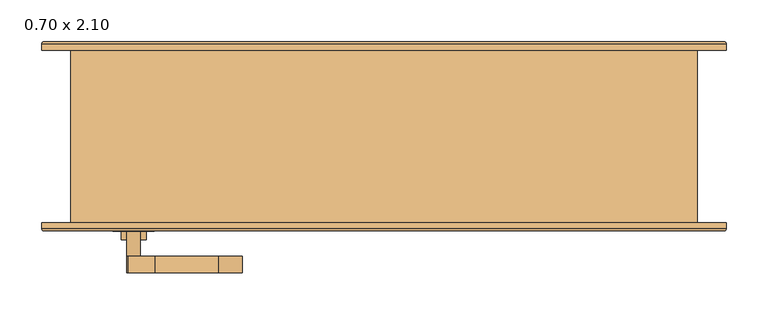
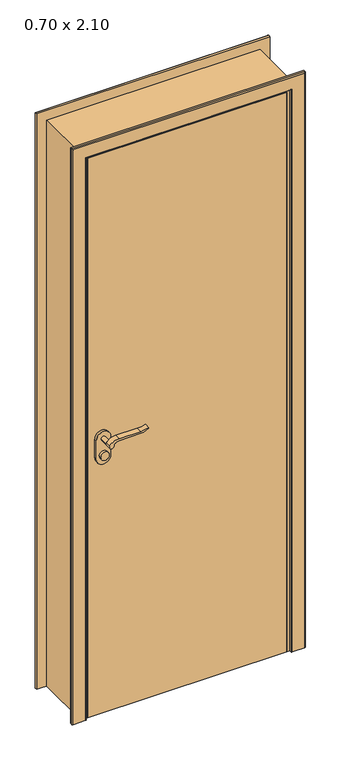
"""IFC4 building model written with IfcOpenShell, lengths in millimetres: door geometry, .CC_ND 300_PORTA SIMPLES DE ABRIR_COM EXTENSÃO : 0.70 x 2.10."""

import ifcopenshell
import ifcopenshell.guid

model = None  # the IFC model being written
_history = None  # IfcOwnerHistory: only IFC2X3 demands one
_inside = {}  # id of a spatial element -> (the spatial element, [elements in it])
_under = {}  # id of a project, library or spatial element -> (it, [spatial elements below it])
_declared = {}  # id of a project -> (the project, [libraries it declares])
_typed = {}  # id of a type object -> (the type object, [elements of that type])
_made_of = {}  # id of a material, layer set ... -> (it, [elements and type objects made of it])


def new_model(schema):
    """Start an empty IFC model of exactly this schema.

    Asked for "IFC4X3", IfcOpenShell would pick the latest addendum, in which some entities
    have other attributes; the version numbers below select the first issue.
    IFC2X3 requires an IfcOwnerHistory on every rooted entity: one is made here for all.
    """
    global model, _history
    if schema == "IFC4X3":
        model = ifcopenshell.file(schema_version=(4, 3, 0, 0))
    else:
        model = ifcopenshell.file(schema=schema)
    _inside.clear()
    _under.clear()
    _declared.clear()
    _typed.clear()
    _made_of.clear()
    _history = None
    if model.schema == "IFC2X3":
        org = make("IfcOrganization", Name="unknown")
        user = make(
            "IfcPersonAndOrganization",
            ThePerson=make("IfcPerson", FamilyName="unknown"),
            TheOrganization=org,
        )
        app = make(
            "IfcApplication",
            ApplicationDeveloper=org,
            Version="unknown",
            ApplicationFullName="unknown",
            ApplicationIdentifier="unknown",
        )
        _history = make(
            "IfcOwnerHistory",
            OwningUser=user,
            OwningApplication=app,
            ChangeAction="ADDED",
            CreationDate=0,
        )
    return model


def make(cls, **values):
    """One entity of the class cls with the attributes given. An attribute that is None is left unset."""
    return model.create_entity(
        cls, **{name: value for name, value in values.items() if value is not None}
    )


def rooted(cls, **values):
    """An entity with a GlobalId (a new one), such as an element, a storey or a relation."""
    return make(cls, GlobalId=ifcopenshell.guid.new(), OwnerHistory=_history, **values)


def si_unit(unit_type, name, prefix=None):
    """IfcSIUnit, for example si_unit("LENGTHUNIT", "METRE", prefix="MILLI")."""
    return make("IfcSIUnit", UnitType=unit_type, Prefix=prefix, Name=name)


def assignment(units):
    """IfcUnitAssignment: the units of a project."""
    return None if units is None else make("IfcUnitAssignment", Units=units)


def point(xyz):
    """IfcCartesianPoint."""
    return None if xyz is None else make("IfcCartesianPoint", Coordinates=xyz)


def direction(xyz):
    """IfcDirection."""
    return None if xyz is None else make("IfcDirection", DirectionRatios=xyz)


def frame(location, z_axis=None, x_axis=None):
    """IfcAxis2Placement3D, a coordinate frame: its origin and axes. An axis left out is left unset."""
    return make(
        "IfcAxis2Placement3D",
        Location=point(location),
        Axis=direction(z_axis),
        RefDirection=direction(x_axis),
    )


def frame_2d(location, x_axis=None):
    """IfcAxis2Placement2D, a coordinate frame in the plane: its origin and x axis."""
    return make(
        "IfcAxis2Placement2D", Location=point(location), RefDirection=direction(x_axis)
    )


def origin():
    """The frame at (0, 0, 0) with its axes left unset."""
    return frame((0.0, 0.0, 0.0))


def origin_with_axes():
    """The frame at (0, 0, 0) with the z axis (0, 0, 1) and the x axis (1, 0, 0) written out."""
    return frame((0.0, 0.0, 0.0), z_axis=(0.0, 0.0, 1.0), x_axis=(1.0, 0.0, 0.0))


def place(relative_to, where):
    """IfcLocalPlacement: puts the frame where relative to a parent placement (None: the world)."""
    return make(
        "IfcLocalPlacement", PlacementRelTo=relative_to, RelativePlacement=where
    )


def context(
    kind, dimensions, precision=None, world=None, true_north=None, identifier=None
):
    """IfcGeometricRepresentationContext, for example the 3D "Model" context."""
    return make(
        "IfcGeometricRepresentationContext",
        ContextIdentifier=identifier,
        ContextType=kind,
        CoordinateSpaceDimension=dimensions,
        Precision=precision,
        WorldCoordinateSystem=world,
        TrueNorth=true_north,
    )


def project(units=None, contexts=None):
    """IfcProject with its units and contexts."""
    return rooted(
        "IfcProject",
        Name="project",
        RepresentationContexts=contexts,
        UnitsInContext=assignment(units),
    )


def spatial(cls, under=None, at=None, **own):
    """A site, building, storey or space (cls), placed at a placement, below another one or the project."""
    s = rooted(cls, ObjectPlacement=at, **own)
    if under is not None:
        _under.setdefault(under.id(), (under, []))[1].append(s)
    return s


def polyline(points):
    """IfcPolyline through the points."""
    return make("IfcPolyline", Points=[point(p) for p in points])


def circle_curve(where, radius):
    """IfcCircle in the frame where."""
    return make("IfcCircle", Position=where, Radius=radius)


def ellipse_curve(where, semi_axis1, semi_axis2):
    """IfcEllipse in the frame where."""
    return make(
        "IfcEllipse", Position=where, SemiAxis1=semi_axis1, SemiAxis2=semi_axis2
    )


def trimmed(basis, trim1, trim2, sense, master):
    """IfcTrimmedCurve: the piece of a basis curve between two trims."""
    return make(
        "IfcTrimmedCurve",
        BasisCurve=basis,
        Trim1=trim1,
        Trim2=trim2,
        SenseAgreement=sense,
        MasterRepresentation=master,
    )


def segment(curve, same_sense, transition):
    """IfcCompositeCurveSegment."""
    return make(
        "IfcCompositeCurveSegment",
        Transition=transition,
        SameSense=same_sense,
        ParentCurve=curve,
    )


def composite_curve(segments, self_intersect=None):
    """IfcCompositeCurve: segments joined end to end."""
    return make("IfcCompositeCurve", Segments=segments, SelfIntersect=self_intersect)


def outline(outer, holes=None, kind="AREA"):
    """IfcArbitraryClosedProfileDef: a profile drawn as a closed curve; with holes, ...WithVoids."""
    if holes is None:
        return make("IfcArbitraryClosedProfileDef", ProfileType=kind, OuterCurve=outer)
    return make(
        "IfcArbitraryProfileDefWithVoids",
        ProfileType=kind,
        OuterCurve=outer,
        InnerCurves=holes,
    )


def extrude(swept, where, along, depth):
    """IfcExtrudedAreaSolid: the profile swept, set in the frame where, extruded along a direction by depth."""
    return make(
        "IfcExtrudedAreaSolid",
        SweptArea=swept,
        Position=where,
        ExtrudedDirection=direction(along),
        Depth=depth,
    )


def faces_of(points, faces, orient=None, outer=None):
    """IfcFace entities. A face is a list of loops; a loop is a list of indices into points, from 0.

    orient and outer hold one flag for each loop. By default every Orientation is true, the
    first loop of a face is its IfcFaceOuterBound and the others are IfcFaceBound.
    """
    made = []
    for i, loops in enumerate(faces):
        bounds = []
        for j, loop in enumerate(loops):
            is_outer = j == 0 if outer is None else outer[i][j]
            bounds.append(
                make(
                    "IfcFaceOuterBound" if is_outer else "IfcFaceBound",
                    Bound=make("IfcPolyLoop", Polygon=[points[k] for k in loop]),
                    Orientation=True if orient is None else orient[i][j],
                )
            )
        made.append(make("IfcFace", Bounds=bounds))
    return made


def faceted_brep(points, faces, orient=None, outer=None, voids=None):
    """IfcFacetedBrep: a solid bounded by flat faces; with voids (closed shells), ...WithVoids."""
    shared = [point(p) for p in points]
    hull = make("IfcClosedShell", CfsFaces=faces_of(shared, faces, orient, outer))
    if voids is None:
        return make("IfcFacetedBrep", Outer=hull)
    return make(
        "IfcFacetedBrepWithVoids",
        Outer=hull,
        Voids=[
            make(cls, CfsFaces=faces_of(shared, fs, o, b)) for cls, fs, o, b in voids
        ],
    )


def shape(context_of_items, identifier, shape_type, items):
    """IfcShapeRepresentation: the items that make up one representation, for example the "Body"."""
    return make(
        "IfcShapeRepresentation",
        ContextOfItems=context_of_items,
        RepresentationIdentifier=identifier,
        RepresentationType=shape_type,
        Items=items,
    )


def source(mapping_origin, context_of_items, identifier, shape_type, items):
    """IfcRepresentationMap: a shape defined once, which mapped items show again and again."""
    return make(
        "IfcRepresentationMap",
        MappingOrigin=mapping_origin,
        MappedRepresentation=shape(context_of_items, identifier, shape_type, items),
    )


def transform(
    local_origin,
    x_axis=None,
    y_axis=None,
    z_axis=None,
    scale=None,
    scale2=None,
    scale3=None,
    uniform=True,
):
    """IfcCartesianTransformationOperator3D, or its non-uniform kind. x_axis, y_axis, z_axis: its Axis1, 2, 3."""
    if uniform:
        return make(
            "IfcCartesianTransformationOperator3D",
            Axis1=direction(x_axis),
            Axis2=direction(y_axis),
            LocalOrigin=point(local_origin),
            Scale=scale,
            Axis3=direction(z_axis),
        )
    return make(
        "IfcCartesianTransformationOperator3DnonUniform",
        Axis1=direction(x_axis),
        Axis2=direction(y_axis),
        LocalOrigin=point(local_origin),
        Scale=scale,
        Axis3=direction(z_axis),
        Scale2=scale2,
        Scale3=scale3,
    )


def mapped(mapping_source, mapping_target):
    """IfcMappedItem: shows the shape of a source again, moved by a transform."""
    return make(
        "IfcMappedItem", MappingSource=mapping_source, MappingTarget=mapping_target
    )


def made_of(thing, what):
    """Note that an element or type object is made of a material, layer set ...; save() writes the relation."""
    if what is not None:
        _made_of.setdefault(what.id(), (what, []))[1].append(thing)
    return thing


def element(
    cls,
    number,
    at=None,
    inside=None,
    cuts=None,
    type_object=None,
    material=None,
    context=None,
    identifier="Body",
    shape_type=None,
    held_by="IfcProductDefinitionShape",
    body=None,
    shapes=None,
    **own,
):
    """One element of the class cls, such as IfcWall. Its Tag is "e" and its number.

    at: its placement. inside: the storey or other place that contains it. cuts: it is an
    opening in that element (IfcRelVoidsElement). A single representation is given by context,
    identifier, shape_type and body (its items); several are given by shapes. held_by: the class
    of the entity that holds the representations. save() writes the other relations.
    """
    e = rooted(cls, Tag="e%d" % number, ObjectPlacement=at, **own)
    if body is not None:
        shapes = [shape(context, identifier, shape_type, body)]
    if shapes is not None:
        e.Representation = make(held_by, Representations=shapes)
    if inside is not None:
        _inside.setdefault(inside.id(), (inside, []))[1].append(e)
    if cuts is not None:
        rooted(
            "IfcRelVoidsElement", RelatingBuildingElement=cuts, RelatedOpeningElement=e
        )
    if type_object is not None:
        _typed.setdefault(type_object.id(), (type_object, []))[1].append(e)
    return made_of(e, material)


def aggregate(whole, parts):
    """IfcRelAggregates: a whole, such as a stair, and the parts it consists of."""
    return rooted("IfcRelAggregates", RelatingObject=whole, RelatedObjects=parts)


def save(model, path):
    """Write the relations noted so far, then the file.

    IfcRelAggregates (storeys below a building ...), IfcRelContainedInSpatialStructure (elements
    in a storey), IfcRelDefinesByType, IfcRelAssociatesMaterial and IfcRelDeclares: one each for
    every whole, place, type object, material and project.
    """
    for whole, parts in _under.values():
        aggregate(whole, parts)
    for where, things in _inside.values():
        rooted(
            "IfcRelContainedInSpatialStructure",
            RelatedElements=things,
            RelatingStructure=where,
        )
    for kind, things in _typed.values():
        rooted("IfcRelDefinesByType", RelatedObjects=things, RelatingType=kind)
    for what, things in _made_of.values():
        rooted("IfcRelAssociatesMaterial", RelatedObjects=things, RelatingMaterial=what)
    for by, libraries in _declared.values():
        rooted("IfcRelDeclares", RelatingContext=by, RelatedDefinitions=libraries)
    model.write(path)


def plane_surface(at):
    """IfcPlane: the flat surface through the origin of the frame at, square to its z axis."""
    return make("IfcPlane", Position=at)


def cylinder_surface(at, radius):
    """IfcCylindricalSurface: all points at the distance radius from the z axis of the frame at."""
    return make("IfcCylindricalSurface", Position=at, Radius=radius)


def advanced_brep(points, edges, surfaces, faces):
    """IfcAdvancedBrep: a solid bounded by faces that lie on surfaces and meet in shared edges.

    An edge is (start, end): straight between two places in points (the first is 0);
    or (start, end, curve); or (start, end, curve, False) where it runs against its curve.
    A face is (place in surfaces, loops), or (place, loops, False) where it looks against
    its surface's normal. A loop lists edges by number (the first is 1), with a minus sign
    where the edge is run from its end to its start. The first loop is the outer one.
    """
    corners = [point(p) for p in points]
    vertices = [make("IfcVertexPoint", VertexGeometry=c) for c in corners]
    made = []
    for start, end, *more in edges:
        made.append(
            make(
                "IfcEdgeCurve",
                EdgeStart=vertices[start],
                EdgeEnd=vertices[end],
                EdgeGeometry=more[0] if more else make("IfcPolyline", Points=[corners[start], corners[end]]),
                SameSense=more[1] if len(more) > 1 else True,
            )
        )
    hull = []
    for where, loops, *sense in faces:
        bounds = []
        for j, loop in enumerate(loops):
            ring = [make("IfcOrientedEdge", EdgeElement=made[abs(k) - 1], Orientation=k > 0) for k in loop]
            bounds.append(
                make(
                    "IfcFaceOuterBound" if j == 0 else "IfcFaceBound",
                    Bound=make("IfcEdgeLoop", EdgeList=ring),
                    Orientation=True,
                )
            )
        hull.append(make("IfcAdvancedFace", Bounds=bounds, FaceSurface=surfaces[where], SameSense=sense[0] if sense else True))
    return make("IfcAdvancedBrep", Outer=make("IfcClosedShell", CfsFaces=hull))


def door_0_70_x_2_10_d125a7d3(model_context):
    return source(origin(), model_context, "Body", "SolidModel", [
        extrude(outline(composite_curve([segment(trimmed(circle_curve(frame_2d((964.5, -300.0)), 15.0), [point((964.5, -285.0))], [point((964.5, -315.0))], False, "CARTESIAN"), True, "CONTINUOUS"), segment(trimmed(circle_curve(frame_2d((964.5, -300.0)), 15.0), [point((964.5, -315.0))], [point((964.5, -285.0))], False, "CARTESIAN"), True, "CONTINUOUS")], self_intersect=False)), frame((0.0, -120.7, 0.0), z_axis=(0.0, 1.0, 0.0), x_axis=(0.0, 0.0, 1.0)), (0.0, 0.0, 1.0), 10.0),
        extrude(outline(composite_curve([segment(trimmed(circle_curve(frame_2d((964.5, -300.0)), 15.0), [point((964.5, -285.0))], [point((964.5, -315.0))], False, "CARTESIAN"), True, "CONTINUOUS"), segment(trimmed(circle_curve(frame_2d((964.5, -300.0)), 15.0), [point((964.5, -315.0))], [point((964.5, -285.0))], False, "CARTESIAN"), True, "CONTINUOUS")], self_intersect=False)), frame((0.0, -60.7, 0.0), z_axis=(0.0, 1.0, 0.0), x_axis=(0.0, 0.0, 1.0)), (0.0, 0.0, 1.0), 10.0),
        extrude(outline(composite_curve([segment(trimmed(circle_curve(frame_2d((1024.5, -300.0)), 8.0), [point((1029.1523287, -306.5081363))], [point((1024.5, -292.0))], False, "CARTESIAN"), True, "CONTINUOUS"), segment(trimmed(circle_curve(frame_2d((1019.3738613, -274.6138099)), 18.1261387), [point((1024.5, -292.0))], [point((1037.5, -274.6138099))], True, "CARTESIAN"), True, "CONTINUOUS"), segment(polyline([(1037.5, -274.6138099), (1037.5, -198.3564091)]), True, "CONTINUOUS"), segment(trimmed(circle_curve(frame_2d((1096.7709207, -201.9396612)), 59.3791355), [point((1037.5, -198.3564091))], [point((1046.7135558, -170.0))], False, "CARTESIAN"), True, "CONTINUOUS"), segment(polyline([(1046.7135558, -170.0), (1049.5, -170.0)]), True, "CONTINUOUS"), segment(trimmed(circle_curve(frame_2d((1127.7850638, -198.4227909)), 83.2850902), [point((1049.5, -170.0))], [point((1044.5, -198.3564091))], True, "CARTESIAN"), True, "CONTINUOUS"), segment(polyline([(1044.5, -198.3564091), (1044.5, -274.6325667)]), True, "CONTINUOUS"), segment(trimmed(circle_curve(frame_2d((1007.2555521, -276.3324871)), 37.2832219), [point((1044.5, -274.6325667))], [point((1029.1523287, -306.5081363))], False, "CARTESIAN"), True, "CONTINUOUS")], self_intersect=False)), frame((0.0, -160.7, 0.0), z_axis=(0.0, 1.0, 0.0), x_axis=(0.0, 0.0, 1.0)), (0.0, 0.0, 1.0), 20.0),
        extrude(outline(composite_curve([segment(trimmed(circle_curve(frame_2d((1019.3738682, -274.6138122)), 18.1261318), [point((1024.4999903, -292.0))], [point((1037.5, -274.6138122))], True, "CARTESIAN"), True, "CONTINUOUS"), segment(polyline([(1037.5, -274.6138122), (1037.5, -198.3564091)]), True, "CONTINUOUS"), segment(trimmed(circle_curve(frame_2d((1096.7709207, -201.9396612)), 59.3791355), [point((1037.5, -198.3564091))], [point((1046.7135558, -170.0))], False, "CARTESIAN"), True, "CONTINUOUS"), segment(polyline([(1046.7135558, -170.0), (1049.5, -170.0)]), True, "CONTINUOUS"), segment(trimmed(circle_curve(frame_2d((1127.7850638, -198.4227909)), 83.2850902), [point((1049.5, -170.0))], [point((1044.5, -198.3564091))], True, "CARTESIAN"), True, "CONTINUOUS"), segment(polyline([(1044.5, -198.3564091), (1044.5, -274.6325667)]), True, "CONTINUOUS"), segment(trimmed(circle_curve(frame_2d((1007.2555521, -276.3324871)), 37.2832219), [point((1044.5, -274.6325667))], [point((1029.1523287, -306.5081363))], False, "CARTESIAN"), True, "CONTINUOUS"), segment(trimmed(circle_curve(frame_2d((1024.5, -300.0)), 8.0), [point((1029.1523287, -306.5081363))], [point((1024.4999903, -292.0))], False, "CARTESIAN"), True, "CONTINUOUS")], self_intersect=False)), frame((0.0, -30.7, 0.0), z_axis=(0.0, 1.0, 0.0), x_axis=(0.0, 0.0, 1.0)), (0.0, 0.0, 1.0), 20.0),
        extrude(outline(composite_curve([segment(trimmed(circle_curve(frame_2d((1024.5, -300.0)), 8.0), [point((1024.5, -292.0))], [point((1024.5, -308.0))], False, "CARTESIAN"), True, "CONTINUOUS"), segment(trimmed(circle_curve(frame_2d((1024.5, -300.0)), 8.0), [point((1024.5, -308.0))], [point((1024.5, -292.0))], False, "CARTESIAN"), True, "CONTINUOUS")], self_intersect=False)), frame((0.0, -140.7, 0.0), z_axis=(0.0, 1.0, 0.0), x_axis=(0.0, 0.0, 1.0)), (0.0, 0.0, 1.0), 30.0),
        extrude(outline(composite_curve([segment(trimmed(circle_curve(frame_2d((1024.5, -300.0)), 8.0), [point((1024.5, -292.0))], [point((1024.5, -308.0))], False, "CARTESIAN"), True, "CONTINUOUS"), segment(trimmed(circle_curve(frame_2d((1024.5, -300.0)), 8.0), [point((1024.5, -308.0))], [point((1024.5, -292.0))], False, "CARTESIAN"), True, "CONTINUOUS")], self_intersect=False)), frame((0.0, -60.7, 0.0), z_axis=(0.0, 1.0, 0.0), x_axis=(0.0, 0.0, 1.0)), (0.0, 0.0, 1.0), 30.0),
        extrude(outline(composite_curve([segment(trimmed(circle_curve(frame_2d((954.5, -300.0)), 25.0), [point((954.5, -325.0))], [point((954.5, -275.0))], False, "CARTESIAN"), True, "CONTINUOUS"), segment(polyline([(954.5, -275.0), (1024.5, -275.0)]), True, "CONTINUOUS"), segment(trimmed(circle_curve(frame_2d((1024.5, -300.0)), 25.0), [point((1024.5, -275.0))], [point((1024.5, -325.0))], False, "CARTESIAN"), True, "CONTINUOUS"), segment(polyline([(1024.5, -325.0), (954.5, -325.0)]), True, "CONTINUOUS")], self_intersect=False)), frame((0.0, -110.7, 0.0), z_axis=(0.0, 1.0, 0.0), x_axis=(0.0, 0.0, 1.0)), (0.0, 0.0, 1.0), 10.0),
        extrude(outline(composite_curve([segment(trimmed(circle_curve(frame_2d((954.5, -300.0)), 25.0), [point((954.5, -325.0))], [point((954.5, -275.0))], False, "CARTESIAN"), True, "CONTINUOUS"), segment(polyline([(954.5, -275.0), (1024.5, -275.0)]), True, "CONTINUOUS"), segment(trimmed(circle_curve(frame_2d((1024.5, -300.0)), 25.0), [point((1024.5, -275.0))], [point((1024.5, -325.0))], False, "CARTESIAN"), True, "CONTINUOUS"), segment(polyline([(1024.5, -325.0), (954.5, -325.0)]), True, "CONTINUOUS")], self_intersect=False)), frame((0.0, -70.7, 0.0), z_axis=(0.0, 1.0, 0.0), x_axis=(0.0, 0.0, 1.0)), (0.0, 0.0, 1.0), 10.0),
        advanced_brep(
        [(-410.0, -100.7, 0.0), (-360.0, -100.7, 0.0), (-360.0, -107.7, 0.0), (-363.0, -110.7, 0.0), (-407.0, -110.7, 0.0), (-410.0, -107.7, 0.0), (-410.0, -100.7, 2135.0), (410.0, -100.7, 2135.0), (410.0, -100.7, 0.0), (360.0, -100.7, 0.0), (360.0, -100.7, 2085.0), (-360.0, -100.7, 2085.0), (-360.0, -107.7, 2085.0), (-363.0, -110.7, 2088.0), (363.0, -110.7, 2088.0), (363.0, -110.7, 0.0), (407.0, -110.7, 0.0), (407.0, -110.7, 2132.0), (-407.0, -110.7, 2132.0), (-410.0, -107.7, 2135.0), (410.0, -107.7, 2135.0), (410.0, -107.7, 0.0), (360.0, -107.7, 0.0), (360.0, -107.7, 2085.0)],
        [
            (0, 1),
            (1, 2),
            (2, 3, circle_curve(frame((-363.0, -107.7, 0.0), z_axis=(0.0, 0.0, -1.0), x_axis=(1.0, 0.0, 0.0)), 3.0)),
            (3, 4),
            (4, 5, circle_curve(frame((-407.0, -107.7, 0.0), z_axis=(0.0, 0.0, -1.0), x_axis=(1.0, 0.0, 0.0)), 3.0)),
            (5, 0),
            (0, 6),
            (6, 7),
            (7, 8),
            (8, 9),
            (9, 10),
            (10, 11),
            (11, 1),
            (11, 12),
            (12, 2),
            (12, 13, ellipse_curve(frame((-363.0, -107.7, 2088.0), z_axis=(-0.7071067811865475, 0.0, -0.7071067811865475), x_axis=(0.7071067811865474, 0.0, -0.7071067811865476)), 4.2426407, 3.0)),
            (13, 3),
            (13, 14),
            (14, 15),
            (15, 16),
            (16, 17),
            (17, 18),
            (18, 4),
            (18, 19, ellipse_curve(frame((-407.0, -107.7, 2132.0), z_axis=(-0.7071067811865475, 0.0, -0.7071067811865475), x_axis=(0.7071067811865474, 0.0, -0.7071067811865476)), 4.2426407, 3.0)),
            (19, 5),
            (19, 6),
            (7, 20),
            (20, 21),
            (21, 8),
            (21, 16, circle_curve(frame((407.0, -107.7, 0.0), z_axis=(0.0, 0.0, -1.0), x_axis=(-1.0, 0.0, 0.0)), 3.0)),
            (15, 22, circle_curve(frame((363.0, -107.7, 0.0), z_axis=(0.0, 0.0, -1.0), x_axis=(-1.0, 0.0, 0.0)), 3.0)),
            (22, 9),
            (23, 10),
            (22, 23),
            (14, 23, ellipse_curve(frame((363.0, -107.7, 2088.0), z_axis=(0.7071067811865475, 0.0, -0.7071067811865475), x_axis=(0.7071067811865474, 0.0, 0.7071067811865476)), 4.2426407, 3.0)),
            (20, 17, ellipse_curve(frame((407.0, -107.7, 2132.0), z_axis=(0.7071067811865475, 0.0, -0.7071067811865475), x_axis=(0.7071067811865474, 0.0, 0.7071067811865476)), 4.2426407, 3.0)),
            (23, 12),
            (19, 20),
        ],
        [
            plane_surface(frame((-360.0, -100.7, 0.0), z_axis=(0.0, 0.0, -1.0), x_axis=(0.0, 1.0, 0.0))),
            plane_surface(frame((-410.0, -100.7, 0.0), z_axis=(0.0, 1.0, 0.0), x_axis=(0.0, 0.0, 1.0))),
            plane_surface(frame((-360.0, -100.7, 0.0), z_axis=(1.0, 0.0, 0.0), x_axis=(0.0, 0.0, 1.0))),
            cylinder_surface(frame((-363.0, -107.7, 0.0), z_axis=(0.0, 0.0, -1.0), x_axis=(1.0, 0.0, 0.0)), 3.0),
            plane_surface(frame((-363.0, -110.7, 0.0), z_axis=(0.0, -1.0, 0.0), x_axis=(0.0, 0.0, 1.0))),
            cylinder_surface(frame((-407.0, -107.7, 0.0), z_axis=(0.0, 0.0, -1.0), x_axis=(1.0, 0.0, 0.0)), 3.0),
            plane_surface(frame((-410.0, -107.7, 0.0), z_axis=(-1.0, 0.0, 0.0), x_axis=(0.0, 0.0, 1.0))),
            plane_surface(frame((410.0, -107.7, 2135.0), z_axis=(1.0, 0.0, 0.0), x_axis=(0.0, 0.0, -1.0))),
            plane_surface(frame((360.0, -100.7, 0.0), z_axis=(0.0, 0.0, -1.0), x_axis=(0.0, 1.0, 0.0))),
            plane_surface(frame((360.0, -100.7, 2085.0), z_axis=(-1.0, 0.0, 0.0), x_axis=(0.0, 0.0, -1.0))),
            cylinder_surface(frame((363.0, -107.7, 2085.0), z_axis=(0.0, 0.0, 1.0), x_axis=(-1.0, 0.0, 0.0)), 3.0),
            cylinder_surface(frame((407.0, -107.7, 2085.0), z_axis=(0.0, 0.0, 1.0), x_axis=(-1.0, 0.0, 0.0)), 3.0),
            plane_surface(frame((-360.0, -100.7, 2085.0), z_axis=(0.0, 0.0, -1.0), x_axis=(1.0, 0.0, 0.0))),
            plane_surface(frame((-410.0, -107.7, 2135.0), z_axis=(0.0, 0.0, 1.0), x_axis=(1.0, 0.0, 0.0))),
            cylinder_surface(frame((-360.0, -107.7, 2088.0), z_axis=(-1.0, 0.0, 0.0), x_axis=(0.0, 0.0, -1.0)), 3.0),
            cylinder_surface(frame((-360.0, -107.7, 2132.0), z_axis=(-1.0, 0.0, 0.0), x_axis=(0.0, 0.0, -1.0)), 3.0),
        ],
        [
            (0, [[1, 2, 3, 4, 5, 6]]),
            (1, [[-1, 7, 8, 9, 10, 11, 12, 13]]),
            (2, [[-2, -13, 14, 15]]),
            (3, [[-3, -15, 16, 17]]),
            (4, [[-4, -17, 18, 19, 20, 21, 22, 23]]),
            (5, [[-5, -23, 24, 25]]),
            (6, [[-6, -25, 26, -7]]),
            (7, [[27, 28, 29, -9]]),
            (8, [[-29, 30, -20, 31, 32, -10]]),
            (9, [[33, -11, -32, 34]]),
            (10, [[35, -34, -31, -19]]),
            (11, [[36, -21, -30, -28]]),
            (12, [[-14, -12, -33, 37]]),
            (13, [[-26, 38, -27, -8]]),
            (14, [[-16, -37, -35, -18]]),
            (15, [[-24, -22, -36, -38]]),
        ],
    ),
        advanced_brep(
        [(410.0, 106.0, 0.0), (360.0, 106.0, 0.0), (360.0, 113.0157283, 0.0), (362.9842717, 116.0, 0.0), (407.0342217, 116.0, 0.0), (410.0, 113.0342217, 0.0), (410.0, 106.0, 2135.0), (-410.0, 106.0, 2135.0), (-410.0, 106.0, 0.0), (-360.0, 106.0, 0.0), (-360.0, 106.0, 2085.0), (360.0, 106.0, 2085.0), (360.0, 113.0157283, 2085.0), (362.9842717, 116.0, 2087.9842717), (-362.9842717, 116.0, 2087.9842717), (-362.9842717, 116.0, 0.0), (-407.0342217, 116.0, 0.0), (-407.0342217, 116.0, 2132.0342217), (407.0342217, 116.0, 2132.0342217), (410.0, 113.0342217, 2135.0), (-410.0, 113.0342217, 2135.0), (-410.0, 113.0342217, 0.0), (-360.0, 113.0157283, 0.0), (-360.0, 113.0157283, 2085.0)],
        [
            (0, 1),
            (1, 2),
            (2, 3, circle_curve(frame((362.9842717, 113.0157283, 0.0), z_axis=(0.0, 0.0, -1.0), x_axis=(1.0, 0.0, 0.0)), 2.9842717)),
            (3, 4),
            (4, 5, circle_curve(frame((407.0342217, 113.0342217, 0.0), z_axis=(0.0, 0.0, -1.0), x_axis=(1.0, 0.0, 0.0)), 2.9657783)),
            (5, 0),
            (0, 6),
            (6, 7),
            (7, 8),
            (8, 9),
            (9, 10),
            (10, 11),
            (11, 1),
            (11, 12),
            (12, 2),
            (12, 13, ellipse_curve(frame((362.9842717, 113.0157283, 2087.9842717), z_axis=(0.7071067811865475, 0.0, -0.7071067811865475), x_axis=(-0.7071067811865474, 0.0, -0.7071067811865476)), 4.2203975, 2.9842717)),
            (13, 3),
            (13, 14),
            (14, 15),
            (15, 16),
            (16, 17),
            (17, 18),
            (18, 4),
            (18, 19, ellipse_curve(frame((407.0342217, 113.0342217, 2132.0342217), z_axis=(0.7071067811865475, 0.0, -0.7071067811865475), x_axis=(-0.7071067811865474, 0.0, -0.7071067811865476)), 4.1942438, 2.9657783)),
            (19, 5),
            (19, 6),
            (7, 20),
            (20, 21),
            (21, 8),
            (21, 16, circle_curve(frame((-407.0342217, 113.0342217, 0.0), z_axis=(0.0, 0.0, -1.0), x_axis=(-1.0, 0.0, 0.0)), 2.9657783)),
            (15, 22, circle_curve(frame((-362.9842717, 113.0157283, 0.0), z_axis=(0.0, 0.0, -1.0), x_axis=(-1.0, 0.0, 0.0)), 2.9842717)),
            (22, 9),
            (23, 10),
            (22, 23),
            (14, 23, ellipse_curve(frame((-362.9842717, 113.0157283, 2087.9842717), z_axis=(-0.7071067811865475, 0.0, -0.7071067811865475), x_axis=(-0.7071067811865474, 0.0, 0.7071067811865476)), 4.2203975, 2.9842717)),
            (20, 17, ellipse_curve(frame((-407.0342217, 113.0342217, 2132.0342217), z_axis=(-0.7071067811865475, 0.0, -0.7071067811865475), x_axis=(-0.7071067811865474, 0.0, 0.7071067811865476)), 4.1942438, 2.9657783)),
            (23, 12),
            (19, 20),
        ],
        [
            plane_surface(frame((360.0, 106.0, 0.0), z_axis=(0.0, 0.0, -1.0), x_axis=(0.0, 1.0, 0.0))),
            plane_surface(frame((410.0, 106.0, 0.0), z_axis=(0.0, -1.0, 0.0), x_axis=(0.0, 0.0, 1.0))),
            plane_surface(frame((360.0, 106.0, 0.0), z_axis=(-1.0, 0.0, 0.0), x_axis=(0.0, 0.0, 1.0))),
            cylinder_surface(frame((362.9842717, 113.0157283, 0.0), z_axis=(0.0, 0.0, -1.0), x_axis=(1.0, 0.0, 0.0)), 2.9842717),
            plane_surface(frame((362.9842717, 116.0, 0.0), z_axis=(0.0, 1.0, 0.0), x_axis=(0.0, 0.0, 1.0))),
            cylinder_surface(frame((407.0342217, 113.0342217, 0.0), z_axis=(0.0, 0.0, -1.0), x_axis=(1.0, 0.0, 0.0)), 2.9657783),
            plane_surface(frame((410.0, 113.0342217, 0.0), z_axis=(1.0, 0.0, 0.0), x_axis=(0.0, 0.0, 1.0))),
            plane_surface(frame((-410.0, 113.0342217, 2135.0), z_axis=(-1.0, 0.0, 0.0), x_axis=(0.0, 0.0, -1.0))),
            plane_surface(frame((-360.0, 106.0, 0.0), z_axis=(0.0, 0.0, -1.0), x_axis=(0.0, 1.0, 0.0))),
            plane_surface(frame((-360.0, 106.0, 2085.0), z_axis=(1.0, 0.0, 0.0), x_axis=(0.0, 0.0, -1.0))),
            cylinder_surface(frame((-362.9842717, 113.0157283, 2085.0), z_axis=(0.0, 0.0, 1.0), x_axis=(-1.0, 0.0, 0.0)), 2.9842717),
            cylinder_surface(frame((-407.0342217, 113.0342217, 2085.0), z_axis=(0.0, 0.0, 1.0), x_axis=(-1.0, 0.0, 0.0)), 2.9657783),
            plane_surface(frame((360.0, 106.0, 2085.0), z_axis=(0.0, 0.0, -1.0), x_axis=(-1.0, 0.0, 0.0))),
            plane_surface(frame((410.0, 113.0342217, 2135.0), z_axis=(0.0, 0.0, 1.0), x_axis=(-1.0, 0.0, 0.0))),
            cylinder_surface(frame((360.0, 113.0157283, 2087.9842717), z_axis=(1.0, 0.0, 0.0), x_axis=(0.0, 0.0, 1.0)), 2.9842717),
            cylinder_surface(frame((360.0, 113.0342217, 2132.0342217), z_axis=(1.0, 0.0, 0.0), x_axis=(0.0, 0.0, 1.0)), 2.9657783),
        ],
        [
            (0, [[1, 2, 3, 4, 5, 6]]),
            (1, [[-1, 7, 8, 9, 10, 11, 12, 13]]),
            (2, [[-2, -13, 14, 15]]),
            (3, [[-3, -15, 16, 17]]),
            (4, [[-4, -17, 18, 19, 20, 21, 22, 23]]),
            (5, [[-5, -23, 24, 25]]),
            (6, [[-6, -25, 26, -7]]),
            (7, [[27, 28, 29, -9]]),
            (8, [[-29, 30, -20, 31, 32, -10]]),
            (9, [[33, -11, -32, 34]]),
            (10, [[35, -34, -31, -19]]),
            (11, [[36, -21, -30, -28]]),
            (12, [[-14, -12, -33, 37]]),
            (13, [[-26, 38, -27, -8]]),
            (14, [[-16, -37, -35, -18]]),
            (15, [[-24, -22, -36, -38]]),
        ],
    ),
        faceted_brep([(342.0, 106.0, 0.0), (375.0, 106.0, 0.0), (375.0, -100.7, 0.0), (350.0, -100.7, 0.0), (350.0, -70.7, 0.0), (342.0, -70.7, 0.0), (342.0, 106.0, 2067.0), (-342.0, 106.0, 2067.0), (-342.0, 106.0, 0.0), (-375.0, 106.0, 0.0), (-375.0, 106.0, 2100.0), (375.0, 106.0, 2100.0), (375.0, -100.7, 2100.0), (-375.0, -100.7, 2100.0), (-375.0, -100.7, 0.0), (-350.0, -100.7, 0.0), (-350.0, -100.7, 2075.0), (350.0, -100.7, 2075.0), (350.0, -70.7, 2075.0), (-350.0, -70.7, 2075.0), (-350.0, -70.7, 0.0), (-342.0, -70.7, 0.0), (-342.0, -70.7, 2067.0), (342.0, -70.7, 2067.0)], [[[0, 1, 2, 3, 4, 5]], [[1, 0, 6, 7, 8, 9, 10, 11]], [[2, 1, 11, 12]], [[3, 2, 12, 13, 14, 15, 16, 17]], [[4, 3, 17, 18]], [[5, 4, 18, 19, 20, 21, 22, 23]], [[0, 5, 23, 6]], [[7, 22, 21, 8]], [[8, 21, 20, 15, 14, 9]], [[13, 10, 9, 14]], [[19, 16, 15, 20]], [[12, 11, 10, 13]], [[18, 17, 16, 19]], [[6, 23, 22, 7]]]),
        extrude(outline(polyline([(-350.0, -70.7), (350.0, -70.7), (350.0, -100.7), (-350.0, -100.7), (-350.0, -70.7)])), origin_with_axes(), (0.0, 0.0, 1.0), 2075.0),
    ])


if __name__ == "__main__":
    model = new_model("IFC4")
    model_context = context("Model", 3, world=origin())
    ifc_project = project(units=[si_unit("LENGTHUNIT", "METRE", prefix="MILLI")], contexts=[model_context])
    site = spatial("IfcSite", under=ifc_project)
    building = spatial("IfcBuilding", under=site)
    placement = place(None, origin())
    door_0_70_x_2_10_shape = door_0_70_x_2_10_d125a7d3(model_context)
    element("IfcDoor", 1, ObjectType=".CC_ND 300_PORTA SIMPLES DE ABRIR_COM EXTENSÃO : 0.70 x 2.10", at=placement, inside=building, context=model_context, shape_type="MappedRepresentation", body=[
        mapped(door_0_70_x_2_10_shape, transform((0.0, 0.0, 0.0), x_axis=(1.0, 0.0, 0.0), y_axis=(0.0, 1.0, 0.0), z_axis=(0.0, 0.0, 1.0))),
    ])
    save(model, "model.ifc")

# Revit data of these elements
# Type ".CC_ND 300_PORTA SIMPLES DE ABRIR_COM EXTENSÃO : 0.70 x 2.10"
#   Type Mark = "155"
#   Rough Width = 0.75 m
#   Espessura moldura externa = 0.01 m
#   Espessura moldura interna = 0.01 m
#   Largura moldura = 0.05 m
#   Extensão acabamento exterior [instance default] = 0.00 m
#   Extensão acabamento interior [instance default] = 0.00 m
#   Espessura batente = 0.025 m
#   Thickness = 0.03 m
#   Altura batente = 2.085 m
#   Aux Arco [instance default] = 0.70 m
#   Rough Height = 2.125 m
#   Height = 2.10 m
#   Width = 0.70 m
#   Moldura interna [instance default] = yes
#   Moldura externa [instance default] = yes
#   Porta = .MADEIRA COM PINTURA ESMALTE BRANCO ACETINADO
#   Moldura = .MADEIRA COM PINTURA ESMALTE BRANCO ACETINADO
#   Maçaneta = .ALUMÍNIO
#   Batente = .MADEIRA COM PINTURA ESMALTE BRANCO ACETINADO
#   Function = (empty or 0)
#   Wall Closure = (empty or 0)
# Element 1 (IfcDoor, ".CC_ND 300_PORTA SIMPLES DE ABRIR_COM EXTENSÃO : 0.70 x 2.10")
#   Extensão acabamento exterior = 0.031 m
#   Extensão acabamento interior = 0.0257 m
#   Aux Arco = 0.7257 m
#   Materials on its faces: ".MADEIRA COM PINTURA ESMALTE BRANCO ACETINADO", ".ALUMÍNIO"
# Materials
#   ".MADEIRA COM PINTURA ESMALTE BRANCO ACETINADO": class ".CC_MADEIRAS", colour RGB 240 240 240, transparency 0, Description = "Madeira com pintura esmalte branco acetinado.", Cost = 0
#   ".ALUMÍNIO": class "CC_METAIS", colour RGB 244 244 244, transparency 0, Description = "Material alumínio", Cost = 0
